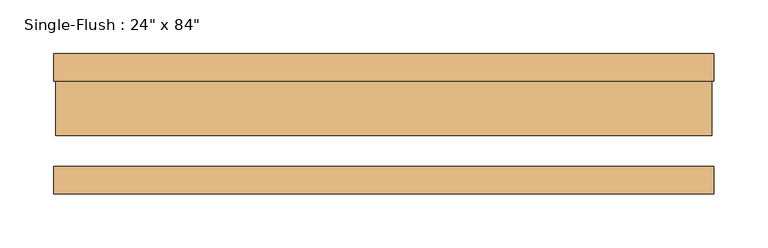
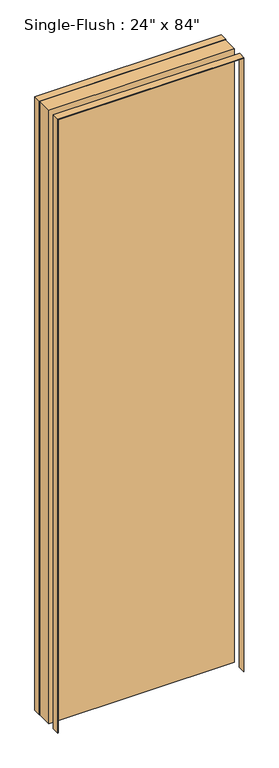
"""IFC4 building model written with IfcOpenShell, lengths in millimetres: door geometry."""

from ifc_helpers import new_model, si_unit, frame, origin, origin_with_axes, place, context, project, spatial, polyline, outline, extrude, source, transform, mapped, element, save


def door_aa2ddddb(model_context):
    return source(origin(), model_context, "Body", "SweptSolid", [
        extrude(outline(polyline([(2135.1875, -306.3875), (0.0, -306.3875), (0.0, -304.8), (2133.6, -304.8), (2133.6, 304.8), (0.0, 304.8), (0.0, 306.3875), (2135.1875, 306.3875), (2135.1875, -306.3875)])), frame((0.0, 39.6875, 0.0), z_axis=(0.0, 1.0, 0.0), x_axis=(0.0, 0.0, 1.0)), (0.0, 0.0, 1.0), 25.4),
        extrude(outline(polyline([(2135.1875, 306.3875), (2135.1875, -306.3875), (0.0, -306.3875), (0.0, -304.8), (2133.6, -304.8), (2133.6, 304.8), (0.0, 304.8), (0.0, 306.3875), (2135.1875, 306.3875)])), frame((0.0, -65.0875, 0.0), z_axis=(0.0, 1.0, 0.0), x_axis=(0.0, 0.0, 1.0)), (0.0, 0.0, 1.0), 25.4),
        extrude(outline(polyline([(304.8, -11.1125), (-304.8, -11.1125), (-304.8, 39.6875), (304.8, 39.6875), (304.8, -11.1125)])), origin_with_axes(), (0.0, 0.0, 1.0), 2133.6),
    ])


if __name__ == "__main__":
    model = new_model("IFC4")
    model_context = context("Model", 3, world=origin())
    ifc_project = project(units=[si_unit("LENGTHUNIT", "METRE", prefix="MILLI")], contexts=[model_context])
    site = spatial("IfcSite", under=ifc_project)
    building = spatial("IfcBuilding", under=site)
    placement = place(None, origin())
    door_shape = door_aa2ddddb(model_context)
    element("IfcDoor", 1, ObjectType="Single-Flush : 24\" x 84\"", at=placement, inside=building, context=model_context, shape_type="MappedRepresentation", body=[
        mapped(door_shape, transform((0.0, 0.0, 0.0), x_axis=(1.0, 0.0, 0.0), y_axis=(0.0, 1.0, 0.0), z_axis=(0.0, 0.0, 1.0))),
    ])
    save(model, "model.ifc")

# Revit data of these elements
# Type "Single-Flush : 24\" x 84\""
#   Type Mark = "34"
#   Assembly Code = "C1020"
#   Thickness = 0' - 2"
#   Height = 7' - 0"
#   Trim Projection Ext = 0' - 1"
#   Trim Projection Int = 0' - 1"
#   Trim Width = 0' - 0 1/16"
#   Width = 2' - 0"
#   Door Material = Door - Panel
#   Frame Material = Door - Frame
#   Function = (empty or 0)
#   Wall Closure = (empty or 0)
# Element 1 (IfcDoor, "Single-Flush : 24\" x 84\"")
#   Materials on its faces: "Door - Frame", "Door - Panel"
# Materials
#   "Door - Panel": class "Wood", colour RGB 210 159 95, transparency 0
#   "Door - Frame": class "Miscellaneous", colour RGB 118 70 51, transparency 0
